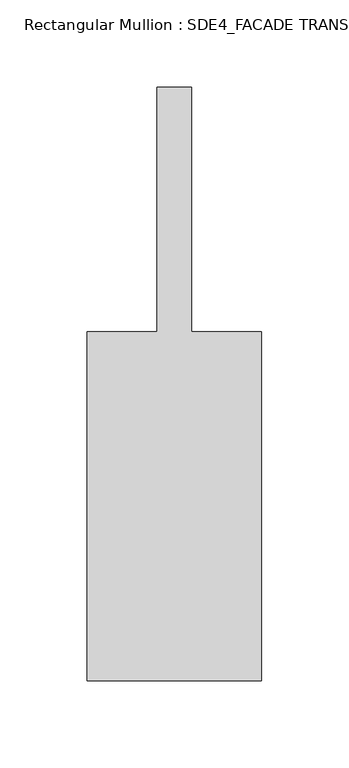
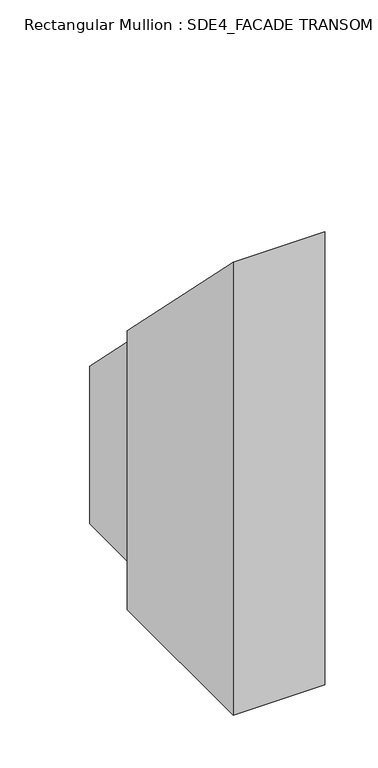
"""IFC4 building model written with IfcOpenShell, lengths in millimetres: member geometry, Rectangular Mullion : SDE4_FACADE TRANSOM TYPE 1."""

import ifcopenshell
import ifcopenshell.guid

model = None  # the IFC model being written
_history = None  # IfcOwnerHistory: only IFC2X3 demands one
_inside = {}  # id of a spatial element -> (the spatial element, [elements in it])
_under = {}  # id of a project, library or spatial element -> (it, [spatial elements below it])
_declared = {}  # id of a project -> (the project, [libraries it declares])
_typed = {}  # id of a type object -> (the type object, [elements of that type])
_made_of = {}  # id of a material, layer set ... -> (it, [elements and type objects made of it])


def new_model(schema):
    """Start an empty IFC model of exactly this schema.

    Asked for "IFC4X3", IfcOpenShell would pick the latest addendum, in which some entities
    have other attributes; the version numbers below select the first issue.
    IFC2X3 requires an IfcOwnerHistory on every rooted entity: one is made here for all.
    """
    global model, _history
    if schema == "IFC4X3":
        model = ifcopenshell.file(schema_version=(4, 3, 0, 0))
    else:
        model = ifcopenshell.file(schema=schema)
    _inside.clear()
    _under.clear()
    _declared.clear()
    _typed.clear()
    _made_of.clear()
    _history = None
    if model.schema == "IFC2X3":
        org = make("IfcOrganization", Name="unknown")
        user = make(
            "IfcPersonAndOrganization",
            ThePerson=make("IfcPerson", FamilyName="unknown"),
            TheOrganization=org,
        )
        app = make(
            "IfcApplication",
            ApplicationDeveloper=org,
            Version="unknown",
            ApplicationFullName="unknown",
            ApplicationIdentifier="unknown",
        )
        _history = make(
            "IfcOwnerHistory",
            OwningUser=user,
            OwningApplication=app,
            ChangeAction="ADDED",
            CreationDate=0,
        )
    return model


def make(cls, **values):
    """One entity of the class cls with the attributes given. An attribute that is None is left unset."""
    return model.create_entity(
        cls, **{name: value for name, value in values.items() if value is not None}
    )


def rooted(cls, **values):
    """An entity with a GlobalId (a new one), such as an element, a storey or a relation."""
    return make(cls, GlobalId=ifcopenshell.guid.new(), OwnerHistory=_history, **values)


def si_unit(unit_type, name, prefix=None):
    """IfcSIUnit, for example si_unit("LENGTHUNIT", "METRE", prefix="MILLI")."""
    return make("IfcSIUnit", UnitType=unit_type, Prefix=prefix, Name=name)


def assignment(units):
    """IfcUnitAssignment: the units of a project."""
    return None if units is None else make("IfcUnitAssignment", Units=units)


def point(xyz):
    """IfcCartesianPoint."""
    return None if xyz is None else make("IfcCartesianPoint", Coordinates=xyz)


def direction(xyz):
    """IfcDirection."""
    return None if xyz is None else make("IfcDirection", DirectionRatios=xyz)


def frame(location, z_axis=None, x_axis=None):
    """IfcAxis2Placement3D, a coordinate frame: its origin and axes. An axis left out is left unset."""
    return make(
        "IfcAxis2Placement3D",
        Location=point(location),
        Axis=direction(z_axis),
        RefDirection=direction(x_axis),
    )


def origin():
    """The frame at (0, 0, 0) with its axes left unset."""
    return frame((0.0, 0.0, 0.0))


def place(relative_to, where):
    """IfcLocalPlacement: puts the frame where relative to a parent placement (None: the world)."""
    return make(
        "IfcLocalPlacement", PlacementRelTo=relative_to, RelativePlacement=where
    )


def context(
    kind, dimensions, precision=None, world=None, true_north=None, identifier=None
):
    """IfcGeometricRepresentationContext, for example the 3D "Model" context."""
    return make(
        "IfcGeometricRepresentationContext",
        ContextIdentifier=identifier,
        ContextType=kind,
        CoordinateSpaceDimension=dimensions,
        Precision=precision,
        WorldCoordinateSystem=world,
        TrueNorth=true_north,
    )


def project(units=None, contexts=None):
    """IfcProject with its units and contexts."""
    return rooted(
        "IfcProject",
        Name="project",
        RepresentationContexts=contexts,
        UnitsInContext=assignment(units),
    )


def spatial(cls, under=None, at=None, **own):
    """A site, building, storey or space (cls), placed at a placement, below another one or the project."""
    s = rooted(cls, ObjectPlacement=at, **own)
    if under is not None:
        _under.setdefault(under.id(), (under, []))[1].append(s)
    return s


def faces_of(points, faces, orient=None, outer=None):
    """IfcFace entities. A face is a list of loops; a loop is a list of indices into points, from 0.

    orient and outer hold one flag for each loop. By default every Orientation is true, the
    first loop of a face is its IfcFaceOuterBound and the others are IfcFaceBound.
    """
    made = []
    for i, loops in enumerate(faces):
        bounds = []
        for j, loop in enumerate(loops):
            is_outer = j == 0 if outer is None else outer[i][j]
            bounds.append(
                make(
                    "IfcFaceOuterBound" if is_outer else "IfcFaceBound",
                    Bound=make("IfcPolyLoop", Polygon=[points[k] for k in loop]),
                    Orientation=True if orient is None else orient[i][j],
                )
            )
        made.append(make("IfcFace", Bounds=bounds))
    return made


def faceted_brep(points, faces, orient=None, outer=None, voids=None):
    """IfcFacetedBrep: a solid bounded by flat faces; with voids (closed shells), ...WithVoids."""
    shared = [point(p) for p in points]
    hull = make("IfcClosedShell", CfsFaces=faces_of(shared, faces, orient, outer))
    if voids is None:
        return make("IfcFacetedBrep", Outer=hull)
    return make(
        "IfcFacetedBrepWithVoids",
        Outer=hull,
        Voids=[
            make(cls, CfsFaces=faces_of(shared, fs, o, b)) for cls, fs, o, b in voids
        ],
    )


def shape(context_of_items, identifier, shape_type, items):
    """IfcShapeRepresentation: the items that make up one representation, for example the "Body"."""
    return make(
        "IfcShapeRepresentation",
        ContextOfItems=context_of_items,
        RepresentationIdentifier=identifier,
        RepresentationType=shape_type,
        Items=items,
    )


def source(mapping_origin, context_of_items, identifier, shape_type, items):
    """IfcRepresentationMap: a shape defined once, which mapped items show again and again."""
    return make(
        "IfcRepresentationMap",
        MappingOrigin=mapping_origin,
        MappedRepresentation=shape(context_of_items, identifier, shape_type, items),
    )


def transform(
    local_origin,
    x_axis=None,
    y_axis=None,
    z_axis=None,
    scale=None,
    scale2=None,
    scale3=None,
    uniform=True,
):
    """IfcCartesianTransformationOperator3D, or its non-uniform kind. x_axis, y_axis, z_axis: its Axis1, 2, 3."""
    if uniform:
        return make(
            "IfcCartesianTransformationOperator3D",
            Axis1=direction(x_axis),
            Axis2=direction(y_axis),
            LocalOrigin=point(local_origin),
            Scale=scale,
            Axis3=direction(z_axis),
        )
    return make(
        "IfcCartesianTransformationOperator3DnonUniform",
        Axis1=direction(x_axis),
        Axis2=direction(y_axis),
        LocalOrigin=point(local_origin),
        Scale=scale,
        Axis3=direction(z_axis),
        Scale2=scale2,
        Scale3=scale3,
    )


def mapped(mapping_source, mapping_target):
    """IfcMappedItem: shows the shape of a source again, moved by a transform."""
    return make(
        "IfcMappedItem", MappingSource=mapping_source, MappingTarget=mapping_target
    )


def made_of(thing, what):
    """Note that an element or type object is made of a material, layer set ...; save() writes the relation."""
    if what is not None:
        _made_of.setdefault(what.id(), (what, []))[1].append(thing)
    return thing


def element(
    cls,
    number,
    at=None,
    inside=None,
    cuts=None,
    type_object=None,
    material=None,
    context=None,
    identifier="Body",
    shape_type=None,
    held_by="IfcProductDefinitionShape",
    body=None,
    shapes=None,
    **own,
):
    """One element of the class cls, such as IfcWall. Its Tag is "e" and its number.

    at: its placement. inside: the storey or other place that contains it. cuts: it is an
    opening in that element (IfcRelVoidsElement). A single representation is given by context,
    identifier, shape_type and body (its items); several are given by shapes. held_by: the class
    of the entity that holds the representations. save() writes the other relations.
    """
    e = rooted(cls, Tag="e%d" % number, ObjectPlacement=at, **own)
    if body is not None:
        shapes = [shape(context, identifier, shape_type, body)]
    if shapes is not None:
        e.Representation = make(held_by, Representations=shapes)
    if inside is not None:
        _inside.setdefault(inside.id(), (inside, []))[1].append(e)
    if cuts is not None:
        rooted(
            "IfcRelVoidsElement", RelatingBuildingElement=cuts, RelatedOpeningElement=e
        )
    if type_object is not None:
        _typed.setdefault(type_object.id(), (type_object, []))[1].append(e)
    return made_of(e, material)


def aggregate(whole, parts):
    """IfcRelAggregates: a whole, such as a stair, and the parts it consists of."""
    return rooted("IfcRelAggregates", RelatingObject=whole, RelatedObjects=parts)


def save(model, path):
    """Write the relations noted so far, then the file.

    IfcRelAggregates (storeys below a building ...), IfcRelContainedInSpatialStructure (elements
    in a storey), IfcRelDefinesByType, IfcRelAssociatesMaterial and IfcRelDeclares: one each for
    every whole, place, type object, material and project.
    """
    for whole, parts in _under.values():
        aggregate(whole, parts)
    for where, things in _inside.values():
        rooted(
            "IfcRelContainedInSpatialStructure",
            RelatedElements=things,
            RelatingStructure=where,
        )
    for kind, things in _typed.values():
        rooted("IfcRelDefinesByType", RelatedObjects=things, RelatingType=kind)
    for what, things in _made_of.values():
        rooted("IfcRelAssociatesMaterial", RelatedObjects=things, RelatingMaterial=what)
    for by, libraries in _declared.values():
        rooted("IfcRelDeclares", RelatingContext=by, RelatedDefinitions=libraries)
    model.write(path)


def rectangular_mullion_sde4_facade_transom_type_1_0e3c8a45(model_context):
    return source(origin(), model_context, "Body", "Brep", [
        faceted_brep([(50.0, -132.5, -389.2348795), (-50.0, -132.5, -389.2348795), (-50.0, 67.5, -389.2348795), (-10.0, 67.5, -389.2348795), (-10.0, 207.5, -389.2348795), (10.0, 207.5, -389.2348795), (10.0, 67.5, -389.2348795), (50.0, 67.5, -389.2348795), (50.0, 67.5, -67.5), (50.0, -132.5, 132.5), (10.0, 67.5, -67.5), (10.0, 207.5, -207.5), (-10.0, 207.5, -207.5), (-10.0, 67.5, -67.5), (-50.0, 67.5, -67.5), (-50.0, -132.5, 132.5)], [[[0, 1, 2, 3, 4, 5, 6, 7]], [[8, 9, 0, 7]], [[10, 8, 7, 6]], [[11, 10, 6, 5]], [[12, 11, 5, 4]], [[13, 12, 4, 3]], [[14, 13, 3, 2]], [[15, 14, 2, 1]], [[9, 15, 1, 0]], [[9, 8, 10, 11, 12, 13, 14, 15]]]),
    ])


if __name__ == "__main__":
    model = new_model("IFC4")
    model_context = context("Model", 3, world=origin())
    ifc_project = project(units=[si_unit("LENGTHUNIT", "METRE", prefix="MILLI")], contexts=[model_context])
    site = spatial("IfcSite", under=ifc_project)
    building = spatial("IfcBuilding", under=site)
    placement = place(None, origin())
    rectangular_mullion_sde4_facade_transom_type_1_shape = rectangular_mullion_sde4_facade_transom_type_1_0e3c8a45(model_context)
    element("IfcMember", 1, ObjectType="Rectangular Mullion : SDE4_FACADE TRANSOM TYPE 1", at=placement, inside=building, context=model_context, shape_type="MappedRepresentation", body=[
        mapped(rectangular_mullion_sde4_facade_transom_type_1_shape, transform((0.0, 0.0, 0.0), x_axis=(1.0, 0.0, 0.0), y_axis=(0.0, 1.0, 0.0), z_axis=(0.0, 0.0, 1.0))),
    ])
    save(model, "model.ifc")

# Revit data of these elements
# Type "Rectangular Mullion : SDE4_FACADE TRANSOM TYPE 1"
#   built-in parameter 1007322 = 1.11549 (stored number, unit not read)
#   built-in parameter 1007321 = 0.164042 (stored number, unit not read)
#   built-in parameter 1007320 = 0.164042 (stored number, unit not read)
